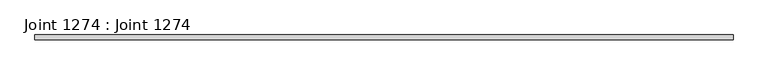
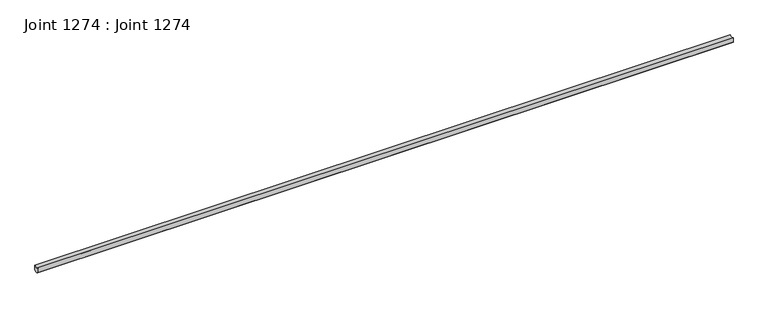
"""IFC4 building model written with IfcOpenShell, lengths in millimetres: proxy geometry, Joint 1274 : Joint 1274."""

from ifc_helpers import new_model, si_unit, point, frame, frame_2d, origin, place, context, project, spatial, polyline, circle_curve, trimmed, segment, composite_curve, outline, extrude, source, transform, mapped, element, save


def joint_1274_joint_1274_0f642f21(model_context):
    return source(origin(), model_context, "Body", "SweptSolid", [
        extrude(outline(composite_curve([segment(polyline([(9744.3002787, 36328.096), (9744.3002787, 36313.846)]), True, "CONTINUOUS"), segment(trimmed(circle_curve(frame_2d((9737.318931, 36320.764173)), 9.8285468), [point((9744.3002787, 36313.846))], [point((9730.3375834, 36313.846))], False, "CARTESIAN"), True, "CONTINUOUS"), segment(polyline([(9730.3375834, 36313.846), (9730.3375834, 36328.096)]), True, "CONTINUOUS"), segment(trimmed(circle_curve(frame_2d((9737.318931, 36335.014173)), 9.8285468), [point((9730.3375834, 36328.096))], [point((9744.3002787, 36328.096))], True, "CARTESIAN"), True, "CONTINUOUS")], self_intersect=False)), frame((3694.2883192, 0.0, 0.0), z_axis=(1.0, 0.0, 0.0), x_axis=(0.0, 1.0, 0.0)), (0.0, 0.0, 1.0), 2000.0),
    ])


if __name__ == "__main__":
    model = new_model("IFC4")
    model_context = context("Model", 3, world=origin())
    ifc_project = project(units=[si_unit("LENGTHUNIT", "METRE", prefix="MILLI")], contexts=[model_context])
    site = spatial("IfcSite", under=ifc_project)
    building = spatial("IfcBuilding", under=site)
    placement = place(None, origin())
    joint_1274_joint_1274_shape = joint_1274_joint_1274_0f642f21(model_context)
    element("IfcBuildingElementProxy", 1, Name="Joint 1274 : Joint 1274", ObjectType="Joint 1274 : Joint 1274", at=placement, inside=building, context=model_context, shape_type="MappedRepresentation", body=[
        mapped(joint_1274_joint_1274_shape, transform((0.0, 0.0, 0.0), x_axis=(1.0, 0.0, 0.0), y_axis=(0.0, 1.0, 0.0), z_axis=(0.0, 0.0, 1.0))),
    ])
    save(model, "model.ifc")

# Revit data of these elements
# Type "Joint 1274 : Joint 1274"
#   NameOverride = "Joint"
# Element 1 (IfcBuildingElementProxy, "Joint 1274 : Joint 1274")
#   Materials on its faces: "SEALANT JOINT"
# Materials
#   "SEALANT JOINT": class "Unassigned", colour RGB 142 225 148, transparency 0
